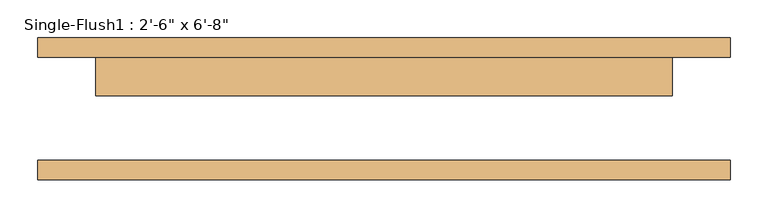
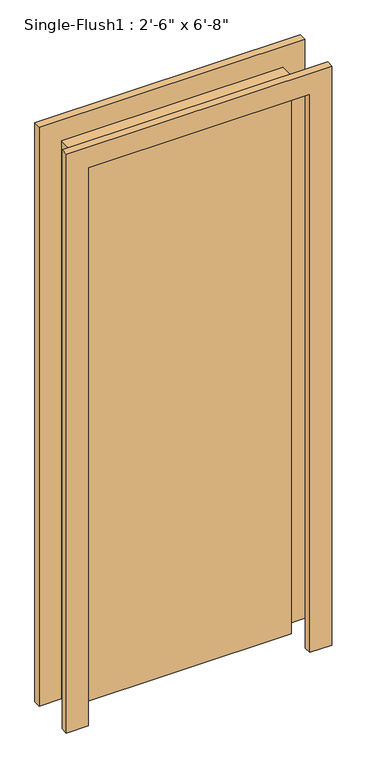
"""IFC4 building model written with IfcOpenShell, lengths in millimetres: door geometry."""

import ifcopenshell
import ifcopenshell.guid

model = None  # the IFC model being written
_history = None  # IfcOwnerHistory: only IFC2X3 demands one
_inside = {}  # id of a spatial element -> (the spatial element, [elements in it])
_under = {}  # id of a project, library or spatial element -> (it, [spatial elements below it])
_declared = {}  # id of a project -> (the project, [libraries it declares])
_typed = {}  # id of a type object -> (the type object, [elements of that type])
_made_of = {}  # id of a material, layer set ... -> (it, [elements and type objects made of it])


def new_model(schema):
    """Start an empty IFC model of exactly this schema.

    Asked for "IFC4X3", IfcOpenShell would pick the latest addendum, in which some entities
    have other attributes; the version numbers below select the first issue.
    IFC2X3 requires an IfcOwnerHistory on every rooted entity: one is made here for all.
    """
    global model, _history
    if schema == "IFC4X3":
        model = ifcopenshell.file(schema_version=(4, 3, 0, 0))
    else:
        model = ifcopenshell.file(schema=schema)
    _inside.clear()
    _under.clear()
    _declared.clear()
    _typed.clear()
    _made_of.clear()
    _history = None
    if model.schema == "IFC2X3":
        org = make("IfcOrganization", Name="unknown")
        user = make(
            "IfcPersonAndOrganization",
            ThePerson=make("IfcPerson", FamilyName="unknown"),
            TheOrganization=org,
        )
        app = make(
            "IfcApplication",
            ApplicationDeveloper=org,
            Version="unknown",
            ApplicationFullName="unknown",
            ApplicationIdentifier="unknown",
        )
        _history = make(
            "IfcOwnerHistory",
            OwningUser=user,
            OwningApplication=app,
            ChangeAction="ADDED",
            CreationDate=0,
        )
    return model


def make(cls, **values):
    """One entity of the class cls with the attributes given. An attribute that is None is left unset."""
    return model.create_entity(
        cls, **{name: value for name, value in values.items() if value is not None}
    )


def rooted(cls, **values):
    """An entity with a GlobalId (a new one), such as an element, a storey or a relation."""
    return make(cls, GlobalId=ifcopenshell.guid.new(), OwnerHistory=_history, **values)


def si_unit(unit_type, name, prefix=None):
    """IfcSIUnit, for example si_unit("LENGTHUNIT", "METRE", prefix="MILLI")."""
    return make("IfcSIUnit", UnitType=unit_type, Prefix=prefix, Name=name)


def assignment(units):
    """IfcUnitAssignment: the units of a project."""
    return None if units is None else make("IfcUnitAssignment", Units=units)


def point(xyz):
    """IfcCartesianPoint."""
    return None if xyz is None else make("IfcCartesianPoint", Coordinates=xyz)


def direction(xyz):
    """IfcDirection."""
    return None if xyz is None else make("IfcDirection", DirectionRatios=xyz)


def frame(location, z_axis=None, x_axis=None):
    """IfcAxis2Placement3D, a coordinate frame: its origin and axes. An axis left out is left unset."""
    return make(
        "IfcAxis2Placement3D",
        Location=point(location),
        Axis=direction(z_axis),
        RefDirection=direction(x_axis),
    )


def origin():
    """The frame at (0, 0, 0) with its axes left unset."""
    return frame((0.0, 0.0, 0.0))


def origin_with_axes():
    """The frame at (0, 0, 0) with the z axis (0, 0, 1) and the x axis (1, 0, 0) written out."""
    return frame((0.0, 0.0, 0.0), z_axis=(0.0, 0.0, 1.0), x_axis=(1.0, 0.0, 0.0))


def place(relative_to, where):
    """IfcLocalPlacement: puts the frame where relative to a parent placement (None: the world)."""
    return make(
        "IfcLocalPlacement", PlacementRelTo=relative_to, RelativePlacement=where
    )


def context(
    kind, dimensions, precision=None, world=None, true_north=None, identifier=None
):
    """IfcGeometricRepresentationContext, for example the 3D "Model" context."""
    return make(
        "IfcGeometricRepresentationContext",
        ContextIdentifier=identifier,
        ContextType=kind,
        CoordinateSpaceDimension=dimensions,
        Precision=precision,
        WorldCoordinateSystem=world,
        TrueNorth=true_north,
    )


def project(units=None, contexts=None):
    """IfcProject with its units and contexts."""
    return rooted(
        "IfcProject",
        Name="project",
        RepresentationContexts=contexts,
        UnitsInContext=assignment(units),
    )


def spatial(cls, under=None, at=None, **own):
    """A site, building, storey or space (cls), placed at a placement, below another one or the project."""
    s = rooted(cls, ObjectPlacement=at, **own)
    if under is not None:
        _under.setdefault(under.id(), (under, []))[1].append(s)
    return s


def polyline(points):
    """IfcPolyline through the points."""
    return make("IfcPolyline", Points=[point(p) for p in points])


def outline(outer, holes=None, kind="AREA"):
    """IfcArbitraryClosedProfileDef: a profile drawn as a closed curve; with holes, ...WithVoids."""
    if holes is None:
        return make("IfcArbitraryClosedProfileDef", ProfileType=kind, OuterCurve=outer)
    return make(
        "IfcArbitraryProfileDefWithVoids",
        ProfileType=kind,
        OuterCurve=outer,
        InnerCurves=holes,
    )


def extrude(swept, where, along, depth):
    """IfcExtrudedAreaSolid: the profile swept, set in the frame where, extruded along a direction by depth."""
    return make(
        "IfcExtrudedAreaSolid",
        SweptArea=swept,
        Position=where,
        ExtrudedDirection=direction(along),
        Depth=depth,
    )


def shape(context_of_items, identifier, shape_type, items):
    """IfcShapeRepresentation: the items that make up one representation, for example the "Body"."""
    return make(
        "IfcShapeRepresentation",
        ContextOfItems=context_of_items,
        RepresentationIdentifier=identifier,
        RepresentationType=shape_type,
        Items=items,
    )


def source(mapping_origin, context_of_items, identifier, shape_type, items):
    """IfcRepresentationMap: a shape defined once, which mapped items show again and again."""
    return make(
        "IfcRepresentationMap",
        MappingOrigin=mapping_origin,
        MappedRepresentation=shape(context_of_items, identifier, shape_type, items),
    )


def transform(
    local_origin,
    x_axis=None,
    y_axis=None,
    z_axis=None,
    scale=None,
    scale2=None,
    scale3=None,
    uniform=True,
):
    """IfcCartesianTransformationOperator3D, or its non-uniform kind. x_axis, y_axis, z_axis: its Axis1, 2, 3."""
    if uniform:
        return make(
            "IfcCartesianTransformationOperator3D",
            Axis1=direction(x_axis),
            Axis2=direction(y_axis),
            LocalOrigin=point(local_origin),
            Scale=scale,
            Axis3=direction(z_axis),
        )
    return make(
        "IfcCartesianTransformationOperator3DnonUniform",
        Axis1=direction(x_axis),
        Axis2=direction(y_axis),
        LocalOrigin=point(local_origin),
        Scale=scale,
        Axis3=direction(z_axis),
        Scale2=scale2,
        Scale3=scale3,
    )


def mapped(mapping_source, mapping_target):
    """IfcMappedItem: shows the shape of a source again, moved by a transform."""
    return make(
        "IfcMappedItem", MappingSource=mapping_source, MappingTarget=mapping_target
    )


def made_of(thing, what):
    """Note that an element or type object is made of a material, layer set ...; save() writes the relation."""
    if what is not None:
        _made_of.setdefault(what.id(), (what, []))[1].append(thing)
    return thing


def element(
    cls,
    number,
    at=None,
    inside=None,
    cuts=None,
    type_object=None,
    material=None,
    context=None,
    identifier="Body",
    shape_type=None,
    held_by="IfcProductDefinitionShape",
    body=None,
    shapes=None,
    **own,
):
    """One element of the class cls, such as IfcWall. Its Tag is "e" and its number.

    at: its placement. inside: the storey or other place that contains it. cuts: it is an
    opening in that element (IfcRelVoidsElement). A single representation is given by context,
    identifier, shape_type and body (its items); several are given by shapes. held_by: the class
    of the entity that holds the representations. save() writes the other relations.
    """
    e = rooted(cls, Tag="e%d" % number, ObjectPlacement=at, **own)
    if body is not None:
        shapes = [shape(context, identifier, shape_type, body)]
    if shapes is not None:
        e.Representation = make(held_by, Representations=shapes)
    if inside is not None:
        _inside.setdefault(inside.id(), (inside, []))[1].append(e)
    if cuts is not None:
        rooted(
            "IfcRelVoidsElement", RelatingBuildingElement=cuts, RelatedOpeningElement=e
        )
    if type_object is not None:
        _typed.setdefault(type_object.id(), (type_object, []))[1].append(e)
    return made_of(e, material)


def aggregate(whole, parts):
    """IfcRelAggregates: a whole, such as a stair, and the parts it consists of."""
    return rooted("IfcRelAggregates", RelatingObject=whole, RelatedObjects=parts)


def save(model, path):
    """Write the relations noted so far, then the file.

    IfcRelAggregates (storeys below a building ...), IfcRelContainedInSpatialStructure (elements
    in a storey), IfcRelDefinesByType, IfcRelAssociatesMaterial and IfcRelDeclares: one each for
    every whole, place, type object, material and project.
    """
    for whole, parts in _under.values():
        aggregate(whole, parts)
    for where, things in _inside.values():
        rooted(
            "IfcRelContainedInSpatialStructure",
            RelatedElements=things,
            RelatingStructure=where,
        )
    for kind, things in _typed.values():
        rooted("IfcRelDefinesByType", RelatedObjects=things, RelatingType=kind)
    for what, things in _made_of.values():
        rooted("IfcRelAssociatesMaterial", RelatedObjects=things, RelatingMaterial=what)
    for by, libraries in _declared.values():
        rooted("IfcRelDeclares", RelatingContext=by, RelatedDefinitions=libraries)
    model.write(path)


def door_0b154108(model_context):
    return source(origin(), model_context, "Body", "SweptSolid", [
        extrude(outline(polyline([(2108.2, -457.2), (0.0, -457.2), (0.0, -381.0), (2032.0, -381.0), (2032.0, 381.0), (0.0, 381.0), (0.0, 457.2), (2108.2, 457.2), (2108.2, -457.2)])), frame((0.0, 68.2625, 0.0), z_axis=(0.0, 1.0, 0.0), x_axis=(0.0, 0.0, 1.0)), (0.0, 0.0, 1.0), 25.4),
        extrude(outline(polyline([(2108.2, 457.2), (2108.2, -457.2), (0.0, -457.2), (0.0, -381.0), (2032.0, -381.0), (2032.0, 381.0), (0.0, 381.0), (0.0, 457.2), (2108.2, 457.2)])), frame((0.0, -93.6625, 0.0), z_axis=(0.0, 1.0, 0.0), x_axis=(0.0, 0.0, 1.0)), (0.0, 0.0, 1.0), 25.4),
        extrude(outline(polyline([(381.0, 17.4625), (-381.0, 17.4625), (-381.0, 68.2625), (381.0, 68.2625), (381.0, 17.4625)])), origin_with_axes(), (0.0, 0.0, 1.0), 2032.0),
    ])


if __name__ == "__main__":
    model = new_model("IFC4")
    model_context = context("Model", 3, world=origin())
    ifc_project = project(units=[si_unit("LENGTHUNIT", "METRE", prefix="MILLI")], contexts=[model_context])
    site = spatial("IfcSite", under=ifc_project)
    building = spatial("IfcBuilding", under=site)
    placement = place(None, origin())
    door_shape = door_0b154108(model_context)
    element("IfcDoor", 1, ObjectType="Single-Flush1 : 2'-6\" x 6'-8\"", at=placement, inside=building, context=model_context, shape_type="MappedRepresentation", body=[
        mapped(door_shape, transform((0.0, 0.0, 0.0), x_axis=(1.0, 0.0, 0.0), y_axis=(0.0, 1.0, 0.0), z_axis=(0.0, 0.0, 1.0))),
    ])
    save(model, "model.ifc")

# Revit data of these elements
# Type "Single-Flush1 : 2'-6\" x 6'-8\""
#   Type Mark = "25"
#   Construction Type Id = "MDOOR"
#   Assembly Code = "C1020"
#   Analytic Construction = "Metal"
#   Thickness = 0' - 2"
#   Heat Transfer Coefficient (U) = 3.7021 W/(m²·K)
#   Height = 6' - 8"
#   Trim Projection Ext = 0' - 1"
#   Trim Projection Int = 0' - 1"
#   Trim Width = 0' - 3"
#   Width = 2' - 6"
#   Door Material = Door - Panel
#   Frame Material = Door - Frame
#   Visual Light Transmittance = 0
#   Solar Heat Gain Coefficient = 0
#   Function = (empty or 0)
#   Wall Closure = (empty or 0)
# Element 1 (IfcDoor, "Single-Flush1 : 2'-6\" x 6'-8\"")
#   Materials on its faces: "Door - Frame", "Door - Panel"
# Materials
#   "Door - Panel": class "Wood", colour RGB 210 159 95, transparency 0, Cost = 0
#   "Door - Frame": class "Miscellaneous", colour RGB 118 70 51, transparency 0, Cost = 0
